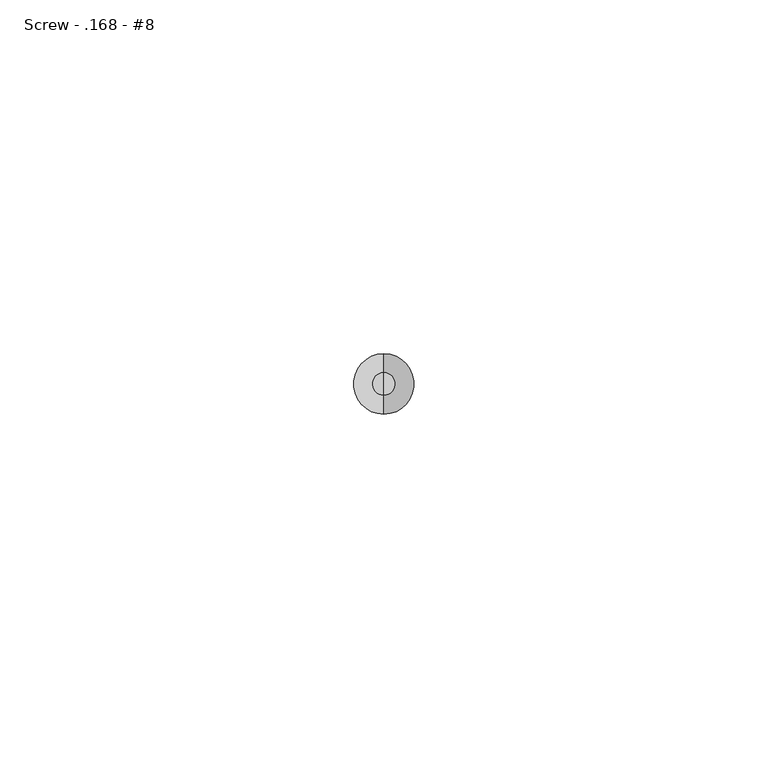
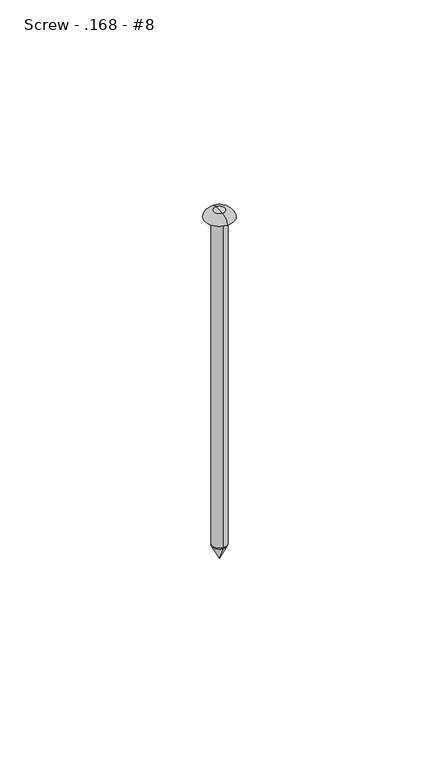
"""IFC4 building model written with IfcOpenShell, lengths in millimetres: fastener geometry, 060523 - W_P_C - Fastenings - Generic : Screw - .168 - #8."""

from ifc_helpers import new_model, si_unit, point, frame, origin, origin_2d, place, context, project, spatial, polyline, circle_curve, ellipse_curve, trimmed, segment, composite_curve, outline, extrude, source, transform, mapped, element, save
from ifc_brep_helpers import plane_surface, revolved_surface, advanced_brep


def screw_168_8_c2f553a8(model_context):
    return source(origin(), model_context, "Body", "SolidModel", [
        advanced_brep(
        [(0.0, -2.1336, -101.6), (0.0, 2.1336, -101.6), (0.0, 0.0, -101.6), (0.0, 0.0, -105.8672)],
        [
            (0, 1, circle_curve(frame((0.0, 0.0, -101.6), z_axis=(0.0, 0.0, 1.0), x_axis=(0.0, 1.0, 0.0)), 2.1336)),
            (1, 2),
            (2, 0),
            (1, 0, circle_curve(frame((0.0, 0.0, -101.6), z_axis=(0.0, 0.0, 1.0), x_axis=(0.0, 1.0, 0.0)), 2.1336)),
            (3, 1),
            (0, 3),
        ],
        [
            plane_surface(frame((0.0, 0.0, -101.6), z_axis=(0.0, 0.0, 1.0), x_axis=(0.0, 1.0, 0.0))),
            revolved_surface(polyline([(0.0, 2.1336, -101.6), (0.0, 0.0, -105.8672)]), (0.0, 0.0, -103.0840259), (0.0, 0.0, -1.0)),
        ],
        [
            (0, [[1, 2, 3]]),
            (0, [[4, -3, -2]]),
            (1, [[5, -1, 6]]),
            (1, [[-6, -4, -5]]),
        ],
    ),
        advanced_brep(
        [(0.0, 4.2672, 0.0), (0.0, -4.2672, 0.0), (0.0, 0.0, 0.0), (0.0, 0.0, 2.1336), (0.0, -1.5875, 2.1336), (0.0, 1.5875, 2.1336)],
        [
            (0, 1, circle_curve(frame((0.0, 0.0, 0.0), z_axis=(0.0, 0.0, -1.0), x_axis=(0.0, -1.0, 0.0)), 4.2672)),
            (1, 2),
            (2, 0),
            (1, 0, circle_curve(frame((0.0, 0.0, 0.0), z_axis=(0.0, 0.0, -1.0), x_axis=(0.0, -1.0, 0.0)), 4.2672)),
            (3, 4),
            (4, 5, circle_curve(frame((0.0, 0.0, 2.1336), z_axis=(0.0, 0.0, 1.0), x_axis=(0.0, -1.0, 0.0)), 1.5875)),
            (5, 3),
            (5, 4, circle_curve(frame((0.0, 0.0, 2.1336), z_axis=(0.0, 0.0, 1.0), x_axis=(0.0, -1.0, 0.0)), 1.5875)),
            (4, 1, circle_curve(frame((0.0, -1.5875, -0.6159878), z_axis=(1.0, 0.0, 0.0), x_axis=(0.0, -1.0, 0.0)), 2.7495878)),
            (0, 5, circle_curve(frame((0.0, 1.5875, -0.6159878), z_axis=(1.0, 0.0, 0.0), x_axis=(0.0, 1.0, 0.0)), 2.7495878)),
        ],
        [
            plane_surface(frame((0.0, 0.0, 0.0), z_axis=(0.0, 0.0, -1.0), x_axis=(0.0, -1.0, 0.0))),
            plane_surface(frame((0.0, 0.0, 2.1336), z_axis=(0.0, 0.0, 1.0), x_axis=(0.0, -1.0, 0.0))),
            revolved_surface(trimmed(ellipse_curve(frame((0.0, -1.5875, -0.6159878), z_axis=(-1.0, 0.0, 0.0), x_axis=(0.0, -1.0, 0.0)), 2.7495878, 2.7495878), [point((0.0, -4.2672, 0.0))], [point((0.0, -1.5875, 2.1336))], True, "CARTESIAN"), (0.0, 0.0, 1.4840259), (0.0, 0.0, 1.0)),
        ],
        [
            (0, [[1, 2, 3]]),
            (0, [[4, -3, -2]]),
            (1, [[5, 6, 7]]),
            (1, [[-7, 8, -5]]),
            (2, [[-6, 9, -1, 10]]),
            (2, [[-8, -10, -4, -9]]),
        ],
    ),
        extrude(outline(composite_curve([segment(trimmed(circle_curve(origin_2d(), 2.1336), [point((0.0, -2.1336))], [point((0.0, 2.1336))], False, "CARTESIAN"), True, "CONTINUOUS"), segment(trimmed(circle_curve(origin_2d(), 2.1336), [point((0.0, 2.1336))], [point((0.0, -2.1336))], False, "CARTESIAN"), True, "CONTINUOUS")], self_intersect=False)), frame((0.0, 0.0, -101.6), z_axis=(0.0, 0.0, 1.0), x_axis=(1.0, 0.0, 0.0)), (0.0, 0.0, 1.0), 101.6),
    ])


if __name__ == "__main__":
    model = new_model("IFC4")
    model_context = context("Model", 3, world=origin())
    ifc_project = project(units=[si_unit("LENGTHUNIT", "METRE", prefix="MILLI")], contexts=[model_context])
    site = spatial("IfcSite", under=ifc_project)
    building = spatial("IfcBuilding", under=site)
    placement = place(None, origin())
    screw_168_8_shape = screw_168_8_c2f553a8(model_context)
    element("IfcFastener", 1, ObjectType="060523 - W_P_C - Fastenings - Generic : Screw - .168 - #8", at=placement, inside=building, context=model_context, shape_type="MappedRepresentation", body=[
        mapped(screw_168_8_shape, transform((0.0, 0.0, 0.0), x_axis=(1.0, 0.0, 0.0), y_axis=(0.0, 1.0, 0.0), z_axis=(0.0, 0.0, 1.0))),
    ])
    save(model, "model.ifc")

# Revit data of these elements
# Type "060523 - W_P_C - Fastenings - Generic : Screw - .168 - #8"
#   Washer_Thickness = 0' - 0.00333"
#   Washer Radius = 0' - 0.094"
#   Washer Offset - Head = 0' - 0"
#   Washer Offset = 0' - 0"
#   Thickness_of_Substrate [instance default] = 0' - 1"
#   Side = 0' - 0 37/64"
#   Radius = 0' - 0.084"
#   Length [instance default] = 0' - 4"
#   Head Size = 0' - 1"
#   Head Radius = 0' - 0 1/2"
#   Head Height = 0' - 0.01"
#   Double Diameter = 0' - 0.336"
#   Diameter = 0' - 0.168"
#   Default Elevation = 4' - 0"
#   Washer_Nut_Visibility = no
#   Washer_Head_Visibility = no
#   Round_Head_Visibility = yes
#   Point Visibility = yes
#   Nut_Visibility = no
#   Hex_Head_Visiblilty = no
#   Washer Material = none
#   Bolt Material (Size) = AT SILL - FASTENER AT 24" O.C.
# Element 1 (IfcFastener, "060523 - W_P_C - Fastenings - Generic : Screw - .168 - #8")
#   Materials on its faces: "AT SILL - FASTENER AT 24\" O.C."
# Materials
#   "AT SILL - FASTENER AT 24\" O.C.": class "Generic", colour RGB 120 120 120, transparency 0, Cost = 0
